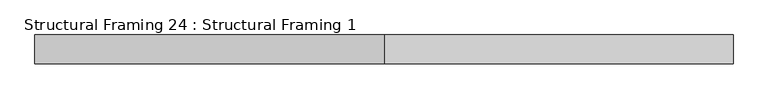
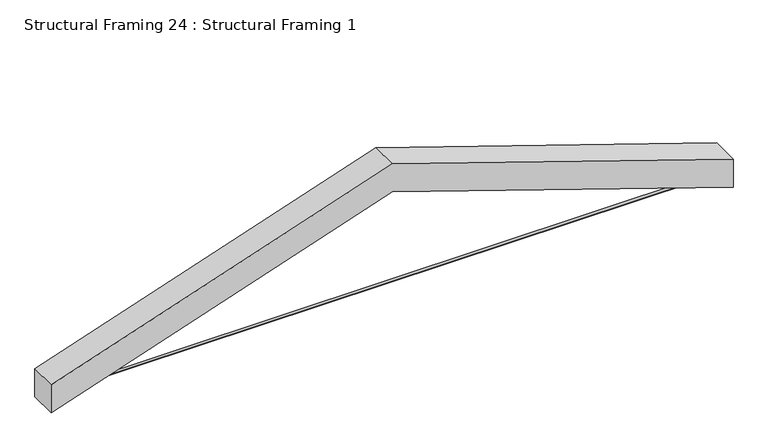
"""IFC4 building model written with IfcOpenShell, lengths in millimetres: beam geometry, Structural Framing 24 : Structural Framing 1."""

from ifc_helpers import new_model, si_unit, point, frame, frame_2d, origin, place, context, project, spatial, polyline, circle_curve, trimmed, segment, composite_curve, outline, extrude, source, transform, mapped, element, save


def structural_framing_24_structural_framing_1_2b149de0(model_context):
    return source(origin(), model_context, "Body", "SweptSolid", [
        extrude(outline(composite_curve([segment(trimmed(circle_curve(frame_2d((2611.1115366, 4984.3019529)), 6.35), [point((2617.4615366, 4984.3019529))], [point((2604.7615366, 4984.3019529))], False, "CARTESIAN"), True, "CONTINUOUS"), segment(trimmed(circle_curve(frame_2d((2611.1115366, 4984.3019529)), 6.35), [point((2604.7615366, 4984.3019529))], [point((2617.4615366, 4984.3019529))], False, "CARTESIAN"), True, "CONTINUOUS")], self_intersect=False)), frame((19888.9870052, 0.0, 0.0), z_axis=(1.0, 0.0, 0.0), x_axis=(0.0, 1.0, 0.0)), (0.0, 0.0, 1.0), 3111.5),
        extrude(outline(polyline([(5652.475838, 21444.7370052), (5084.8528105, 19749.2870052), (4937.5315162, 19749.2870052), (5505.1545437, 21444.7370052), (4937.5315162, 23140.1870052), (5084.8528105, 23140.1870052), (5652.475838, 21444.7370052)])), frame((0.0, 2541.2615366, 0.0), z_axis=(0.0, 1.0, 0.0), x_axis=(0.0, 0.0, 1.0)), (0.0, 0.0, 1.0), 139.7),
    ])


if __name__ == "__main__":
    model = new_model("IFC4")
    model_context = context("Model", 3, world=origin())
    ifc_project = project(units=[si_unit("LENGTHUNIT", "METRE", prefix="MILLI")], contexts=[model_context])
    site = spatial("IfcSite", under=ifc_project)
    building = spatial("IfcBuilding", under=site)
    placement = place(None, origin())
    structural_framing_24_structural_framing_1_shape = structural_framing_24_structural_framing_1_2b149de0(model_context)
    element("IfcBeam", 1, ObjectType="Structural Framing 24 : Structural Framing 1", at=placement, inside=building, context=model_context, shape_type="MappedRepresentation", body=[
        mapped(structural_framing_24_structural_framing_1_shape, transform((0.0, 0.0, 0.0), x_axis=(1.0, 0.0, 0.0), y_axis=(0.0, 1.0, 0.0), z_axis=(0.0, 0.0, 1.0))),
    ])
    save(model, "model.ifc")

# Revit data of these elements
# Element 1 (IfcBeam, "Structural Framing 24 : Structural Framing 1")
#   Materials on its faces: "GLULAM TRUSS W/ CUSTOM GUSSET PLATES", "COLLAR TIE: 1/2\" GALV. ROD"
# Materials
#   "GLULAM TRUSS W/ CUSTOM GUSSET PLATES": class "Generic", colour RGB 206 153 90, transparency 0, Cost = 0
#   "COLLAR TIE: 1/2\" GALV. ROD": class "Generic", colour RGB 49 49 49, transparency 0, Cost = 0
